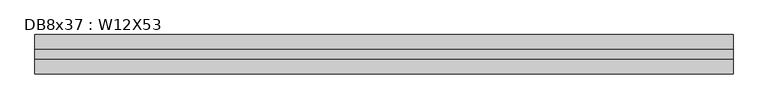
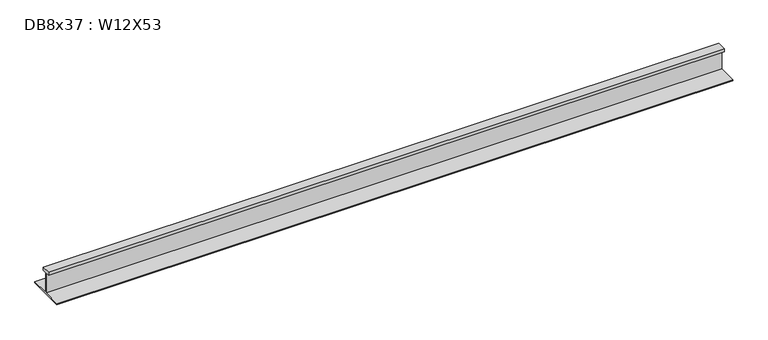
"""IFC4 building model written with IfcOpenShell, lengths in millimetres: beam geometry, DB8x37 : W12X53."""

import ifcopenshell
import ifcopenshell.guid

model = None  # the IFC model being written
_history = None  # IfcOwnerHistory: only IFC2X3 demands one
_inside = {}  # id of a spatial element -> (the spatial element, [elements in it])
_under = {}  # id of a project, library or spatial element -> (it, [spatial elements below it])
_declared = {}  # id of a project -> (the project, [libraries it declares])
_typed = {}  # id of a type object -> (the type object, [elements of that type])
_made_of = {}  # id of a material, layer set ... -> (it, [elements and type objects made of it])


def new_model(schema):
    """Start an empty IFC model of exactly this schema.

    Asked for "IFC4X3", IfcOpenShell would pick the latest addendum, in which some entities
    have other attributes; the version numbers below select the first issue.
    IFC2X3 requires an IfcOwnerHistory on every rooted entity: one is made here for all.
    """
    global model, _history
    if schema == "IFC4X3":
        model = ifcopenshell.file(schema_version=(4, 3, 0, 0))
    else:
        model = ifcopenshell.file(schema=schema)
    _inside.clear()
    _under.clear()
    _declared.clear()
    _typed.clear()
    _made_of.clear()
    _history = None
    if model.schema == "IFC2X3":
        org = make("IfcOrganization", Name="unknown")
        user = make(
            "IfcPersonAndOrganization",
            ThePerson=make("IfcPerson", FamilyName="unknown"),
            TheOrganization=org,
        )
        app = make(
            "IfcApplication",
            ApplicationDeveloper=org,
            Version="unknown",
            ApplicationFullName="unknown",
            ApplicationIdentifier="unknown",
        )
        _history = make(
            "IfcOwnerHistory",
            OwningUser=user,
            OwningApplication=app,
            ChangeAction="ADDED",
            CreationDate=0,
        )
    return model


def make(cls, **values):
    """One entity of the class cls with the attributes given. An attribute that is None is left unset."""
    return model.create_entity(
        cls, **{name: value for name, value in values.items() if value is not None}
    )


def rooted(cls, **values):
    """An entity with a GlobalId (a new one), such as an element, a storey or a relation."""
    return make(cls, GlobalId=ifcopenshell.guid.new(), OwnerHistory=_history, **values)


def si_unit(unit_type, name, prefix=None):
    """IfcSIUnit, for example si_unit("LENGTHUNIT", "METRE", prefix="MILLI")."""
    return make("IfcSIUnit", UnitType=unit_type, Prefix=prefix, Name=name)


def assignment(units):
    """IfcUnitAssignment: the units of a project."""
    return None if units is None else make("IfcUnitAssignment", Units=units)


def point(xyz):
    """IfcCartesianPoint."""
    return None if xyz is None else make("IfcCartesianPoint", Coordinates=xyz)


def direction(xyz):
    """IfcDirection."""
    return None if xyz is None else make("IfcDirection", DirectionRatios=xyz)


def frame(location, z_axis=None, x_axis=None):
    """IfcAxis2Placement3D, a coordinate frame: its origin and axes. An axis left out is left unset."""
    return make(
        "IfcAxis2Placement3D",
        Location=point(location),
        Axis=direction(z_axis),
        RefDirection=direction(x_axis),
    )


def origin():
    """The frame at (0, 0, 0) with its axes left unset."""
    return frame((0.0, 0.0, 0.0))


def place(relative_to, where):
    """IfcLocalPlacement: puts the frame where relative to a parent placement (None: the world)."""
    return make(
        "IfcLocalPlacement", PlacementRelTo=relative_to, RelativePlacement=where
    )


def context(
    kind, dimensions, precision=None, world=None, true_north=None, identifier=None
):
    """IfcGeometricRepresentationContext, for example the 3D "Model" context."""
    return make(
        "IfcGeometricRepresentationContext",
        ContextIdentifier=identifier,
        ContextType=kind,
        CoordinateSpaceDimension=dimensions,
        Precision=precision,
        WorldCoordinateSystem=world,
        TrueNorth=true_north,
    )


def project(units=None, contexts=None):
    """IfcProject with its units and contexts."""
    return rooted(
        "IfcProject",
        Name="project",
        RepresentationContexts=contexts,
        UnitsInContext=assignment(units),
    )


def spatial(cls, under=None, at=None, **own):
    """A site, building, storey or space (cls), placed at a placement, below another one or the project."""
    s = rooted(cls, ObjectPlacement=at, **own)
    if under is not None:
        _under.setdefault(under.id(), (under, []))[1].append(s)
    return s


def polyline(points):
    """IfcPolyline through the points."""
    return make("IfcPolyline", Points=[point(p) for p in points])


def outline(outer, holes=None, kind="AREA"):
    """IfcArbitraryClosedProfileDef: a profile drawn as a closed curve; with holes, ...WithVoids."""
    if holes is None:
        return make("IfcArbitraryClosedProfileDef", ProfileType=kind, OuterCurve=outer)
    return make(
        "IfcArbitraryProfileDefWithVoids",
        ProfileType=kind,
        OuterCurve=outer,
        InnerCurves=holes,
    )


def extrude(swept, where, along, depth):
    """IfcExtrudedAreaSolid: the profile swept, set in the frame where, extruded along a direction by depth."""
    return make(
        "IfcExtrudedAreaSolid",
        SweptArea=swept,
        Position=where,
        ExtrudedDirection=direction(along),
        Depth=depth,
    )


def shape(context_of_items, identifier, shape_type, items):
    """IfcShapeRepresentation: the items that make up one representation, for example the "Body"."""
    return make(
        "IfcShapeRepresentation",
        ContextOfItems=context_of_items,
        RepresentationIdentifier=identifier,
        RepresentationType=shape_type,
        Items=items,
    )


def source(mapping_origin, context_of_items, identifier, shape_type, items):
    """IfcRepresentationMap: a shape defined once, which mapped items show again and again."""
    return make(
        "IfcRepresentationMap",
        MappingOrigin=mapping_origin,
        MappedRepresentation=shape(context_of_items, identifier, shape_type, items),
    )


def transform(
    local_origin,
    x_axis=None,
    y_axis=None,
    z_axis=None,
    scale=None,
    scale2=None,
    scale3=None,
    uniform=True,
):
    """IfcCartesianTransformationOperator3D, or its non-uniform kind. x_axis, y_axis, z_axis: its Axis1, 2, 3."""
    if uniform:
        return make(
            "IfcCartesianTransformationOperator3D",
            Axis1=direction(x_axis),
            Axis2=direction(y_axis),
            LocalOrigin=point(local_origin),
            Scale=scale,
            Axis3=direction(z_axis),
        )
    return make(
        "IfcCartesianTransformationOperator3DnonUniform",
        Axis1=direction(x_axis),
        Axis2=direction(y_axis),
        LocalOrigin=point(local_origin),
        Scale=scale,
        Axis3=direction(z_axis),
        Scale2=scale2,
        Scale3=scale3,
    )


def mapped(mapping_source, mapping_target):
    """IfcMappedItem: shows the shape of a source again, moved by a transform."""
    return make(
        "IfcMappedItem", MappingSource=mapping_source, MappingTarget=mapping_target
    )


def made_of(thing, what):
    """Note that an element or type object is made of a material, layer set ...; save() writes the relation."""
    if what is not None:
        _made_of.setdefault(what.id(), (what, []))[1].append(thing)
    return thing


def element(
    cls,
    number,
    at=None,
    inside=None,
    cuts=None,
    type_object=None,
    material=None,
    context=None,
    identifier="Body",
    shape_type=None,
    held_by="IfcProductDefinitionShape",
    body=None,
    shapes=None,
    **own,
):
    """One element of the class cls, such as IfcWall. Its Tag is "e" and its number.

    at: its placement. inside: the storey or other place that contains it. cuts: it is an
    opening in that element (IfcRelVoidsElement). A single representation is given by context,
    identifier, shape_type and body (its items); several are given by shapes. held_by: the class
    of the entity that holds the representations. save() writes the other relations.
    """
    e = rooted(cls, Tag="e%d" % number, ObjectPlacement=at, **own)
    if body is not None:
        shapes = [shape(context, identifier, shape_type, body)]
    if shapes is not None:
        e.Representation = make(held_by, Representations=shapes)
    if inside is not None:
        _inside.setdefault(inside.id(), (inside, []))[1].append(e)
    if cuts is not None:
        rooted(
            "IfcRelVoidsElement", RelatingBuildingElement=cuts, RelatedOpeningElement=e
        )
    if type_object is not None:
        _typed.setdefault(type_object.id(), (type_object, []))[1].append(e)
    return made_of(e, material)


def aggregate(whole, parts):
    """IfcRelAggregates: a whole, such as a stair, and the parts it consists of."""
    return rooted("IfcRelAggregates", RelatingObject=whole, RelatedObjects=parts)


def save(model, path):
    """Write the relations noted so far, then the file.

    IfcRelAggregates (storeys below a building ...), IfcRelContainedInSpatialStructure (elements
    in a storey), IfcRelDefinesByType, IfcRelAssociatesMaterial and IfcRelDeclares: one each for
    every whole, place, type object, material and project.
    """
    for whole, parts in _under.values():
        aggregate(whole, parts)
    for where, things in _inside.values():
        rooted(
            "IfcRelContainedInSpatialStructure",
            RelatedElements=things,
            RelatingStructure=where,
        )
    for kind, things in _typed.values():
        rooted("IfcRelDefinesByType", RelatedObjects=things, RelatingType=kind)
    for what, things in _made_of.values():
        rooted("IfcRelAssociatesMaterial", RelatedObjects=things, RelatingMaterial=what)
    for by, libraries in _declared.values():
        rooted("IfcRelDeclares", RelatingContext=by, RelatedDefinitions=libraries)
    model.write(path)


def db8x37_w12x53_4241ae81(model_context):
    return source(origin(), model_context, "Body", "SweptSolid", [
        extrude(outline(polyline([(38.1, 145.415), (38.1, 120.015), (2.921, 120.015), (2.921, -48.4505), (152.4, -48.4505), (152.4, -58.1025), (-152.4, -58.1025), (-152.4, -48.4505), (-2.921, -48.4505), (-2.921, 120.015), (-38.1, 120.015), (-38.1, 145.415), (38.1, 145.415)])), frame((-2708.529, 0.0, 0.0), z_axis=(1.0, 0.0, 0.0), x_axis=(0.0, 1.0, 0.0)), (0.0, 0.0, 1.0), 5417.058),
    ])


if __name__ == "__main__":
    model = new_model("IFC4")
    model_context = context("Model", 3, world=origin())
    ifc_project = project(units=[si_unit("LENGTHUNIT", "METRE", prefix="MILLI")], contexts=[model_context])
    site = spatial("IfcSite", under=ifc_project)
    building = spatial("IfcBuilding", under=site)
    placement = place(None, origin())
    db8x37_w12x53_shape = db8x37_w12x53_4241ae81(model_context)
    element("IfcBeam", 1, ObjectType="DB8x37 : W12X53", at=placement, inside=building, context=model_context, shape_type="MappedRepresentation", body=[
        mapped(db8x37_w12x53_shape, transform((0.0, 0.0, 0.0), x_axis=(1.0, 0.0, 0.0), y_axis=(0.0, 1.0, 0.0), z_axis=(0.0, 0.0, 1.0))),
    ])
    save(model, "model.ifc")

# Revit data of these elements
# Type "DB8x37 : W12X53"
#   Assembly Code = "B10"
#   W = 53
#   Length [instance default] = 5' - 0"
#   bf = 0' - 10"
#   d = 1' - 0.1"
#   k = 0' - 1 3/8"
#   k2 = 0' - 0.8"
#   tf = 0' - 0.575"
#   tw = 0' - 0.345"
#   A = 0.108333 SF
#   Structural Material [instance default] = Steel ASTM A992
# Element 1 (IfcBeam, "DB8x37 : W12X53")
#   Materials on its faces: "Steel ASTM A992"
# Materials
#   "Steel ASTM A992": class "Metal", colour RGB 199 199 199, transparency 0, Description = "Structural steel 50ksi", Cost = 0
